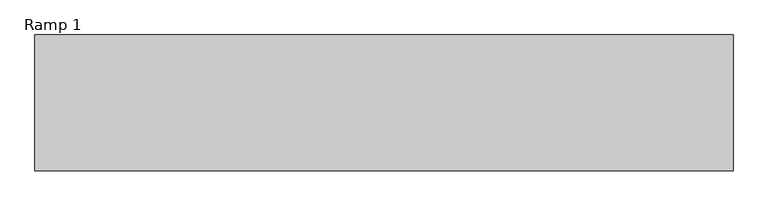
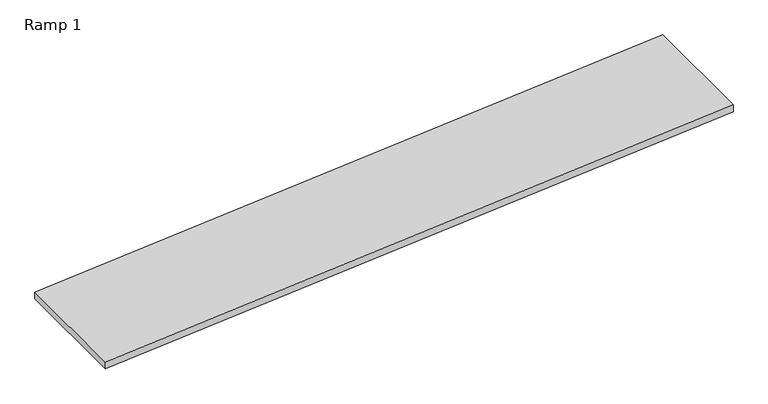
"""IFC4 building model written with IfcOpenShell, lengths in millimetres: ramp geometry, Ramp 1."""

from ifc_helpers import new_model, si_unit, frame, origin, place, context, project, spatial, polyline, outline, extrude, source, transform, mapped, element, save


def ramp_1_6e3daf5e(model_context):
    return source(origin(), model_context, "Body", "SweptSolid", [
        extrude(outline(polyline([(300.0, 60716.32048), (-1200.0, 42716.32048), (-1400.693243, 42716.32048), (99.306757, 60716.32048), (300.0, 60716.32048)])), frame((0.0, 67977.0208589, 0.0), z_axis=(0.0, 1.0, 0.0), x_axis=(0.0, 0.0, 1.0)), (0.0, 0.0, 1.0), 3500.0),
    ])


if __name__ == "__main__":
    model = new_model("IFC4")
    model_context = context("Model", 3, world=origin())
    ifc_project = project(units=[si_unit("LENGTHUNIT", "METRE", prefix="MILLI")], contexts=[model_context])
    site = spatial("IfcSite", under=ifc_project)
    building = spatial("IfcBuilding", under=site)
    placement = place(None, origin())
    ramp_1_shape = ramp_1_6e3daf5e(model_context)
    element("IfcRamp", 1, ObjectType="Ramp 1", at=placement, inside=building, context=model_context, shape_type="MappedRepresentation", body=[
        mapped(ramp_1_shape, transform((0.0, 0.0, 0.0), x_axis=(1.0, 0.0, 0.0), y_axis=(0.0, 1.0, 0.0), z_axis=(0.0, 0.0, 1.0))),
    ])
    save(model, "model.ifc")
